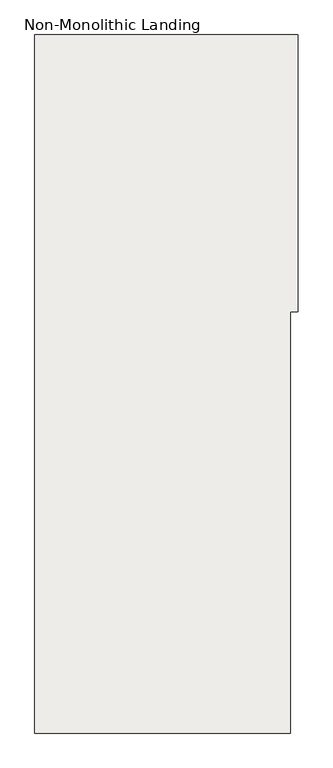
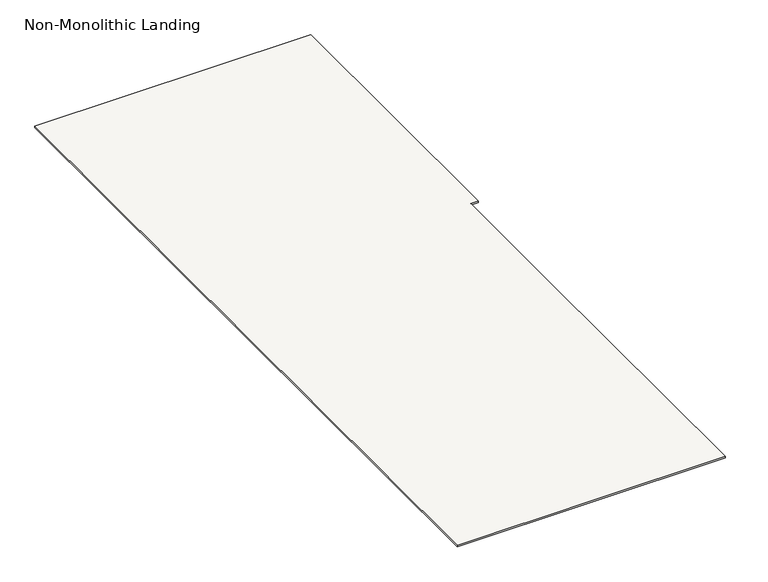
"""IFC4 building model written with IfcOpenShell, lengths in millimetres: slab geometry, Non-Monolithic Landing."""

from ifc_helpers import new_model, si_unit, origin, place, context, project, spatial, faceted_brep, source, transform, mapped, element, save


def non_monolithic_landing_752ad253(model_context):
    return source(origin(), model_context, "Body", "Brep", [
        faceted_brep([(-16318.9400908, 12030.4345331, 18411.7647059), (-16318.0900908, 12030.4345331, 18405.7647059), (-16318.0900908, 13220.4345331, 18405.7647059), (-16318.9400908, 13220.4345331, 18411.7647059), (-16350.0, 11470.4345331, 18411.7647059), (-16350.0, 12030.4345331, 18411.7647059), (-16350.0, 13220.4345331, 18411.7647059), (-17450.0, 13220.4345331, 18411.7647059), (-17450.0, 10220.4345331, 18411.7647059), (-16350.0, 10220.4345331, 18411.7647059), (-16350.0, 12030.4345331, 18405.7647059), (-16350.0, 11470.4345331, 18405.7647059), (-16350.85, 11470.4345331, 18405.7647059), (-16350.85, 10220.4345331, 18405.7647059), (-17450.0, 10220.4345331, 18405.7647059), (-17450.0, 13220.4345331, 18405.7647059), (-16350.0, 13220.4345331, 18405.7647059)], [[[0, 1, 2, 3]], [[4, 5, 0, 3, 6, 7, 8, 9]], [[10, 11, 12, 13, 14, 15, 16, 2, 1]], [[5, 4, 11, 10]], [[0, 5, 10, 1]], [[6, 3, 2, 16]], [[7, 6, 16, 15]], [[8, 7, 15, 14]], [[9, 8, 14, 13]], [[4, 12, 11]], [[12, 4, 9, 13]]]),
    ])


if __name__ == "__main__":
    model = new_model("IFC4")
    model_context = context("Model", 3, world=origin())
    ifc_project = project(units=[si_unit("LENGTHUNIT", "METRE", prefix="MILLI")], contexts=[model_context])
    site = spatial("IfcSite", under=ifc_project)
    building = spatial("IfcBuilding", under=site)
    placement = place(None, origin())
    non_monolithic_landing_shape = non_monolithic_landing_752ad253(model_context)
    element("IfcSlab", 1, ObjectType="Non-Monolithic Landing", at=placement, inside=building, context=model_context, shape_type="MappedRepresentation", body=[
        mapped(non_monolithic_landing_shape, transform((0.0, 0.0, 0.0), x_axis=(1.0, 0.0, 0.0), y_axis=(0.0, 1.0, 0.0), z_axis=(0.0, 0.0, 1.0))),
    ])
    save(model, "model.ifc")

# Revit data of these elements
# Element 1 (IfcSlab, "Non-Monolithic Landing")
#   Materials on its faces: "Steel, Paint Finish, Dark Gray"
# Materials
#   "Steel, Paint Finish, Dark Gray": class "Metal", colour RGB 89 89 89, transparency 0, Description = "Steel, paint finish, dark gray, glossy", Cost = 0
